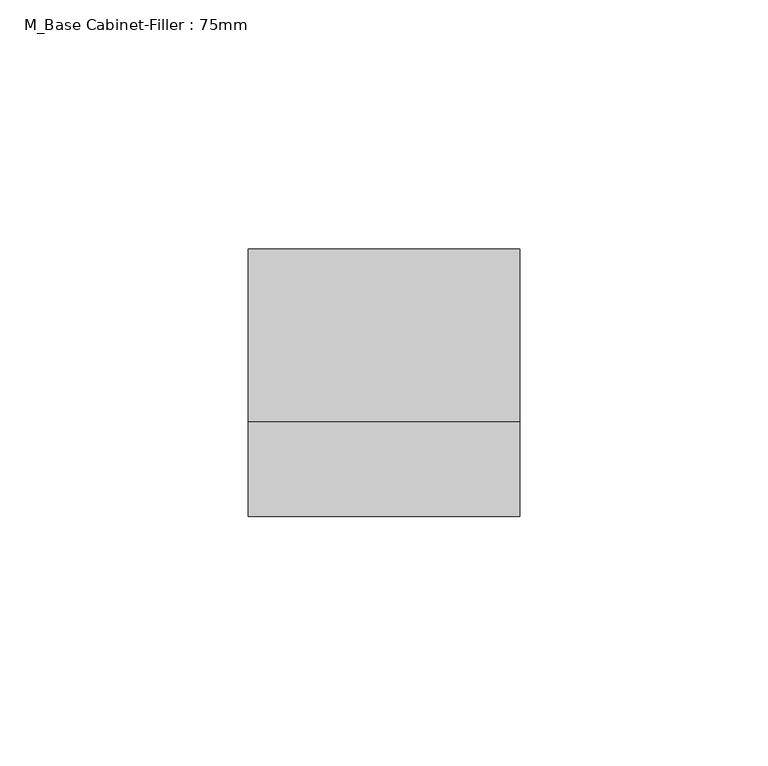
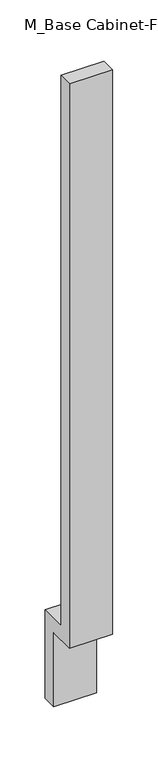
"""IFC4 building model written with IfcOpenShell, lengths in millimetres: furniture geometry, M_Base Cabinet-Filler : 75mm."""

import ifcopenshell
import ifcopenshell.guid

model = None  # the IFC model being written
_history = None  # IfcOwnerHistory: only IFC2X3 demands one
_inside = {}  # id of a spatial element -> (the spatial element, [elements in it])
_under = {}  # id of a project, library or spatial element -> (it, [spatial elements below it])
_declared = {}  # id of a project -> (the project, [libraries it declares])
_typed = {}  # id of a type object -> (the type object, [elements of that type])
_made_of = {}  # id of a material, layer set ... -> (it, [elements and type objects made of it])


def new_model(schema):
    """Start an empty IFC model of exactly this schema.

    Asked for "IFC4X3", IfcOpenShell would pick the latest addendum, in which some entities
    have other attributes; the version numbers below select the first issue.
    IFC2X3 requires an IfcOwnerHistory on every rooted entity: one is made here for all.
    """
    global model, _history
    if schema == "IFC4X3":
        model = ifcopenshell.file(schema_version=(4, 3, 0, 0))
    else:
        model = ifcopenshell.file(schema=schema)
    _inside.clear()
    _under.clear()
    _declared.clear()
    _typed.clear()
    _made_of.clear()
    _history = None
    if model.schema == "IFC2X3":
        org = make("IfcOrganization", Name="unknown")
        user = make(
            "IfcPersonAndOrganization",
            ThePerson=make("IfcPerson", FamilyName="unknown"),
            TheOrganization=org,
        )
        app = make(
            "IfcApplication",
            ApplicationDeveloper=org,
            Version="unknown",
            ApplicationFullName="unknown",
            ApplicationIdentifier="unknown",
        )
        _history = make(
            "IfcOwnerHistory",
            OwningUser=user,
            OwningApplication=app,
            ChangeAction="ADDED",
            CreationDate=0,
        )
    return model


def make(cls, **values):
    """One entity of the class cls with the attributes given. An attribute that is None is left unset."""
    return model.create_entity(
        cls, **{name: value for name, value in values.items() if value is not None}
    )


def rooted(cls, **values):
    """An entity with a GlobalId (a new one), such as an element, a storey or a relation."""
    return make(cls, GlobalId=ifcopenshell.guid.new(), OwnerHistory=_history, **values)


def si_unit(unit_type, name, prefix=None):
    """IfcSIUnit, for example si_unit("LENGTHUNIT", "METRE", prefix="MILLI")."""
    return make("IfcSIUnit", UnitType=unit_type, Prefix=prefix, Name=name)


def assignment(units):
    """IfcUnitAssignment: the units of a project."""
    return None if units is None else make("IfcUnitAssignment", Units=units)


def point(xyz):
    """IfcCartesianPoint."""
    return None if xyz is None else make("IfcCartesianPoint", Coordinates=xyz)


def direction(xyz):
    """IfcDirection."""
    return None if xyz is None else make("IfcDirection", DirectionRatios=xyz)


def frame(location, z_axis=None, x_axis=None):
    """IfcAxis2Placement3D, a coordinate frame: its origin and axes. An axis left out is left unset."""
    return make(
        "IfcAxis2Placement3D",
        Location=point(location),
        Axis=direction(z_axis),
        RefDirection=direction(x_axis),
    )


def origin():
    """The frame at (0, 0, 0) with its axes left unset."""
    return frame((0.0, 0.0, 0.0))


def place(relative_to, where):
    """IfcLocalPlacement: puts the frame where relative to a parent placement (None: the world)."""
    return make(
        "IfcLocalPlacement", PlacementRelTo=relative_to, RelativePlacement=where
    )


def context(
    kind, dimensions, precision=None, world=None, true_north=None, identifier=None
):
    """IfcGeometricRepresentationContext, for example the 3D "Model" context."""
    return make(
        "IfcGeometricRepresentationContext",
        ContextIdentifier=identifier,
        ContextType=kind,
        CoordinateSpaceDimension=dimensions,
        Precision=precision,
        WorldCoordinateSystem=world,
        TrueNorth=true_north,
    )


def project(units=None, contexts=None):
    """IfcProject with its units and contexts."""
    return rooted(
        "IfcProject",
        Name="project",
        RepresentationContexts=contexts,
        UnitsInContext=assignment(units),
    )


def spatial(cls, under=None, at=None, **own):
    """A site, building, storey or space (cls), placed at a placement, below another one or the project."""
    s = rooted(cls, ObjectPlacement=at, **own)
    if under is not None:
        _under.setdefault(under.id(), (under, []))[1].append(s)
    return s


def polyline(points):
    """IfcPolyline through the points."""
    return make("IfcPolyline", Points=[point(p) for p in points])


def outline(outer, holes=None, kind="AREA"):
    """IfcArbitraryClosedProfileDef: a profile drawn as a closed curve; with holes, ...WithVoids."""
    if holes is None:
        return make("IfcArbitraryClosedProfileDef", ProfileType=kind, OuterCurve=outer)
    return make(
        "IfcArbitraryProfileDefWithVoids",
        ProfileType=kind,
        OuterCurve=outer,
        InnerCurves=holes,
    )


def extrude(swept, where, along, depth):
    """IfcExtrudedAreaSolid: the profile swept, set in the frame where, extruded along a direction by depth."""
    return make(
        "IfcExtrudedAreaSolid",
        SweptArea=swept,
        Position=where,
        ExtrudedDirection=direction(along),
        Depth=depth,
    )


def shape(context_of_items, identifier, shape_type, items):
    """IfcShapeRepresentation: the items that make up one representation, for example the "Body"."""
    return make(
        "IfcShapeRepresentation",
        ContextOfItems=context_of_items,
        RepresentationIdentifier=identifier,
        RepresentationType=shape_type,
        Items=items,
    )


def source(mapping_origin, context_of_items, identifier, shape_type, items):
    """IfcRepresentationMap: a shape defined once, which mapped items show again and again."""
    return make(
        "IfcRepresentationMap",
        MappingOrigin=mapping_origin,
        MappedRepresentation=shape(context_of_items, identifier, shape_type, items),
    )


def transform(
    local_origin,
    x_axis=None,
    y_axis=None,
    z_axis=None,
    scale=None,
    scale2=None,
    scale3=None,
    uniform=True,
):
    """IfcCartesianTransformationOperator3D, or its non-uniform kind. x_axis, y_axis, z_axis: its Axis1, 2, 3."""
    if uniform:
        return make(
            "IfcCartesianTransformationOperator3D",
            Axis1=direction(x_axis),
            Axis2=direction(y_axis),
            LocalOrigin=point(local_origin),
            Scale=scale,
            Axis3=direction(z_axis),
        )
    return make(
        "IfcCartesianTransformationOperator3DnonUniform",
        Axis1=direction(x_axis),
        Axis2=direction(y_axis),
        LocalOrigin=point(local_origin),
        Scale=scale,
        Axis3=direction(z_axis),
        Scale2=scale2,
        Scale3=scale3,
    )


def mapped(mapping_source, mapping_target):
    """IfcMappedItem: shows the shape of a source again, moved by a transform."""
    return make(
        "IfcMappedItem", MappingSource=mapping_source, MappingTarget=mapping_target
    )


def made_of(thing, what):
    """Note that an element or type object is made of a material, layer set ...; save() writes the relation."""
    if what is not None:
        _made_of.setdefault(what.id(), (what, []))[1].append(thing)
    return thing


def element(
    cls,
    number,
    at=None,
    inside=None,
    cuts=None,
    type_object=None,
    material=None,
    context=None,
    identifier="Body",
    shape_type=None,
    held_by="IfcProductDefinitionShape",
    body=None,
    shapes=None,
    **own,
):
    """One element of the class cls, such as IfcWall. Its Tag is "e" and its number.

    at: its placement. inside: the storey or other place that contains it. cuts: it is an
    opening in that element (IfcRelVoidsElement). A single representation is given by context,
    identifier, shape_type and body (its items); several are given by shapes. held_by: the class
    of the entity that holds the representations. save() writes the other relations.
    """
    e = rooted(cls, Tag="e%d" % number, ObjectPlacement=at, **own)
    if body is not None:
        shapes = [shape(context, identifier, shape_type, body)]
    if shapes is not None:
        e.Representation = make(held_by, Representations=shapes)
    if inside is not None:
        _inside.setdefault(inside.id(), (inside, []))[1].append(e)
    if cuts is not None:
        rooted(
            "IfcRelVoidsElement", RelatingBuildingElement=cuts, RelatedOpeningElement=e
        )
    if type_object is not None:
        _typed.setdefault(type_object.id(), (type_object, []))[1].append(e)
    return made_of(e, material)


def aggregate(whole, parts):
    """IfcRelAggregates: a whole, such as a stair, and the parts it consists of."""
    return rooted("IfcRelAggregates", RelatingObject=whole, RelatedObjects=parts)


def save(model, path):
    """Write the relations noted so far, then the file.

    IfcRelAggregates (storeys below a building ...), IfcRelContainedInSpatialStructure (elements
    in a storey), IfcRelDefinesByType, IfcRelAssociatesMaterial and IfcRelDeclares: one each for
    every whole, place, type object, material and project.
    """
    for whole, parts in _under.values():
        aggregate(whole, parts)
    for where, things in _inside.values():
        rooted(
            "IfcRelContainedInSpatialStructure",
            RelatedElements=things,
            RelatingStructure=where,
        )
    for kind, things in _typed.values():
        rooted("IfcRelDefinesByType", RelatedObjects=things, RelatingType=kind)
    for what, things in _made_of.values():
        rooted("IfcRelAssociatesMaterial", RelatedObjects=things, RelatingMaterial=what)
    for by, libraries in _declared.values():
        rooted("IfcRelDeclares", RelatingContext=by, RelatedDefinitions=libraries)
    model.write(path)


def m_base_cabinet_filler_75mm_578fa602(model_context):
    return source(origin(), model_context, "Body", "SweptSolid", [
        extrude(outline(polyline([(-600.0, 100.0), (-600.0, 860.0), (-580.95, 860.0), (-580.95, 119.05), (-545.95, 119.05), (-545.95, 0.0), (-565.0, 0.0), (-565.0, 100.0), (-600.0, 100.0)])), frame((-8.5622951, 0.0, 0.0), z_axis=(1.0, 0.0, 0.0), x_axis=(0.0, 1.0, 0.0)), (0.0, 0.0, 1.0), 54.6),
    ])


if __name__ == "__main__":
    model = new_model("IFC4")
    model_context = context("Model", 3, world=origin())
    ifc_project = project(units=[si_unit("LENGTHUNIT", "METRE", prefix="MILLI")], contexts=[model_context])
    site = spatial("IfcSite", under=ifc_project)
    building = spatial("IfcBuilding", under=site)
    placement = place(None, origin())
    m_base_cabinet_filler_75mm_shape = m_base_cabinet_filler_75mm_578fa602(model_context)
    element("IfcFurniture", 1, ObjectType="M_Base Cabinet-Filler : 75mm", at=placement, inside=building, context=model_context, shape_type="MappedRepresentation", body=[
        mapped(m_base_cabinet_filler_75mm_shape, transform((0.0, 0.0, 0.0), x_axis=(1.0, 0.0, 0.0), y_axis=(0.0, 1.0, 0.0), z_axis=(0.0, 0.0, 1.0))),
    ])
    save(model, "model.ifc")

# Revit data of these elements
# Type "M_Base Cabinet-Filler : 75mm"
#   Keynote = "12700"
#   Model = "Hamptons"
#   Manufacturer = "Newcastel Design"
#   Description = "Base Cabinet - Filler"
#   Type Mark = "Base Cabinet 75 mm"
#   COBie.Type.CreatedBy = "design@eagle.com"
#   COBie.Type.CreatedOn = "2016-09-01T06:50:21"
#   COBie.Type.Name = "Casework_M_Base Cabinet-Filler_75mm"
#   COBie.Type.Category = "23-40 35 17 47 11 : Kitchen Casework"
#   COBie.Type.Description = "Base Cabinet - Filler"
#   COBie.Type.Manufacturer = "Newcastel Design"
#   COBie.Type.ModelNumber = "Hamptons"
#   COBie.Type.ReplacementCost = 0
#   Depth = 600 mm
#   Height = 860 mm
#   Plinth Depth = 35 mm
#   Plinth Height = 100 mm
#   Width [instance default] = 75 mm
#   COBie.Type = no
#   Cabinet Material = none
# Element 1 (IfcFurniture, "M_Base Cabinet-Filler : 75mm")
#   Width = 54.6 mm
#   Materials on its faces: "Cabinets"
# Materials
#   "Cabinets": class "Miscellaneous", colour RGB 249 249 249, transparency 0
